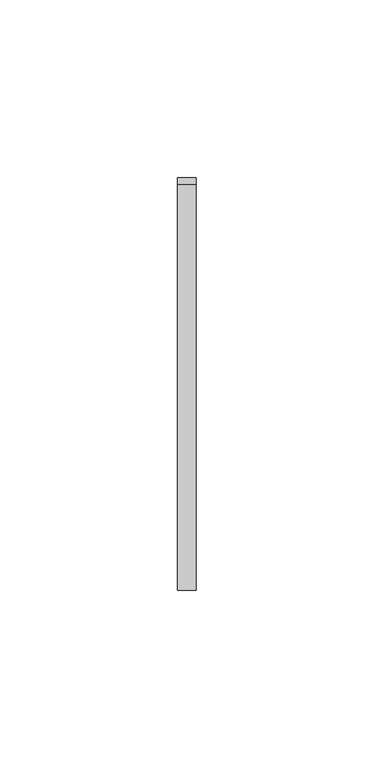
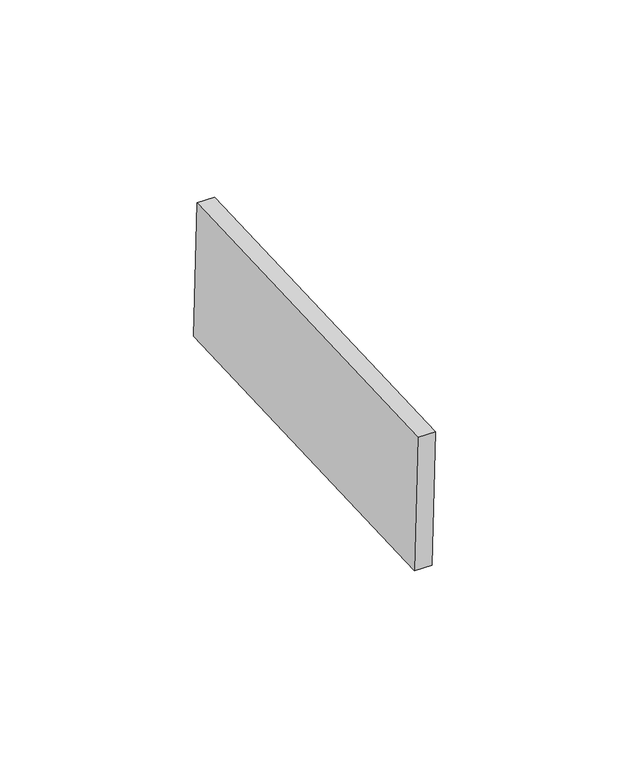
"""IFC4 building model written with IfcOpenShell, lengths in millimetres: proxy geometry, Inner panel:Inner panel:1:Inner panel:1 : Inner panel:Inner panel:300324:2:Inner panel:1:Inner panel:1 : Inner panel:Inner panel:300324:2 : Inner panel:Inner panel:1:Inner panel:1 : Inner panel:Inner panel:300324:300043:90 : Inner panel:Inner panel:1:Inner panel:1 : Inner panel:Inner panel:300324:2:Inner panel:1:Inner panel:1 : Inner panel:Inner panel:300324:2 : Inner panel:Inner panel:1:Inner panel:1 : Inner panel:Inner panel:300324:300043:308120."""

from ifc_helpers import new_model, si_unit, frame, origin, place, context, project, spatial, polyline, outline, extrude, source, transform, mapped, element, save


def generic_models_65679f36(model_context):
    return source(origin(), model_context, "Body", "SweptSolid", [
        extrude(outline(polyline([(0.0, -114.2999999), (0.0, 0.0), (5.2138089, 0.0), (5.2138089, -114.2999999), (0.0, -114.2999999)])), frame((592310.995117, -568168.273882, 8806.9397902), z_axis=(0.0, -0.04163054471215927, 0.9991330730923529), x_axis=(-1.0, 0.0, 0.0)), (0.0, 0.0, 1.0), 43.2233908),
    ])


if __name__ == "__main__":
    model = new_model("IFC4")
    model_context = context("Model", 3, world=origin())
    ifc_project = project(units=[si_unit("LENGTHUNIT", "METRE", prefix="MILLI")], contexts=[model_context])
    site = spatial("IfcSite", under=ifc_project)
    building = spatial("IfcBuilding", under=site)
    placement = place(None, origin())
    generic_models_shape = generic_models_65679f36(model_context)
    element("IfcBuildingElementProxy", 1, Name="Inner panel:Inner panel:1:Inner panel:1 : Inner panel:Inner panel:300324:2:Inner panel:1:Inner panel:1 : Inner panel:Inner panel:300324:2 : Inner panel:Inner panel:1:Inner panel:1 : Inner panel:Inner panel:300324:300043:90 : Inner panel:Inner panel:1:Inner panel:1 : Inner panel:Inner panel:300324:2:Inner panel:1:Inner panel:1 : Inner panel:Inner panel:300324:2 : Inner panel:Inner panel:1:Inner panel:1 : Inner panel:Inner panel:300324:300043:308120", ObjectType="Inner panel:Inner panel:1:Inner panel:1 : Inner panel:Inner panel:300324:2:Inner panel:1:Inner panel:1 : Inner panel:Inner panel:300324:2 : Inner panel:Inner panel:1:Inner panel:1 : Inner panel:Inner panel:300324:300043:90 : Inner panel:Inner panel:1:Inner panel:1 : Inner panel:Inner panel:300324:2:Inner panel:1:Inner panel:1 : Inner panel:Inner panel:300324:2 : Inner panel:Inner panel:1:Inner panel:1 : Inner panel:Inner panel:300324:300043:308120", at=placement, inside=building, context=model_context, shape_type="MappedRepresentation", body=[
        mapped(generic_models_shape, transform((0.0, 0.0, 0.0), x_axis=(1.0, 0.0, 0.0), y_axis=(0.0, 1.0, 0.0), z_axis=(0.0, 0.0, 1.0))),
    ])
    save(model, "model.ifc")

# Revit data of these elements
# Type "Inner panel:Inner panel:1:Inner panel:1 : Inner panel:Inner panel:300324:2:Inner panel:1:Inner panel:1 : Inner panel:Inner panel:300324:2 : Inner panel:Inner panel:1:Inner panel:1 : Inner panel:Inner panel:300324:300043:90 : Inner panel:Inner panel:1:Inner panel:1 : Inner panel:Inner panel:300324:2:Inner panel:1:Inner panel:1 : Inner panel:Inner panel:300324:2 : Inner panel:Inner panel:1:Inner panel:1 : Inner panel:Inner panel:300324:300043:308120"
#   NameOverride = "Inner panel:Inner panel:1:Inner panel:1 : Inner panel:Inner panel:300324:2:Inner panel:1:Inner panel:1 : Inner panel:Inner panel:300324:2 : Inner panel:Inner panel:1:Inner panel:1 : Inner panel:Inner panel:300324:300043:308120"
#   ObjectTypeOverride = "Inner panel:1:Inner panel:1 : Inner panel:Inner panel:300324:2 : Inner panel:Inner panel:1:Inner panel:1 : Inner panel:Inner panel:300324:300043"
#   Reference = "Inner panel"
#   Tag = "308120"
# Element 1 (IfcBuildingElementProxy, "Inner panel:Inner panel:1:Inner panel:1 : Inner panel:Inner panel:300324:2:Inner panel:1:Inner panel:1 : Inner panel:Inner panel:300324:2 : Inner panel:Inner panel:1:Inner panel:1 : Inner panel:Inner panel:300324:300043:90 : Inner panel:Inner panel:1:Inner panel:1 : Inner panel:Inner panel:300324:2:Inner panel:1:Inner panel:1 : Inner panel:Inner panel:300324:2 : Inner panel:Inner panel:1:Inner panel:1 : Inner panel:Inner panel:300324:300043:308120")
#   Materials on its faces: "SLIDING CLIP"
# Materials
#   "SLIDING CLIP": class "Generic", colour RGB 120 120 120, transparency 0, Cost = 0
